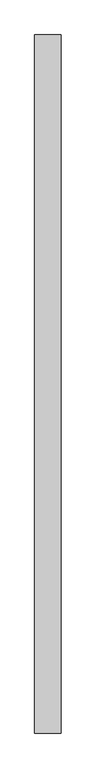
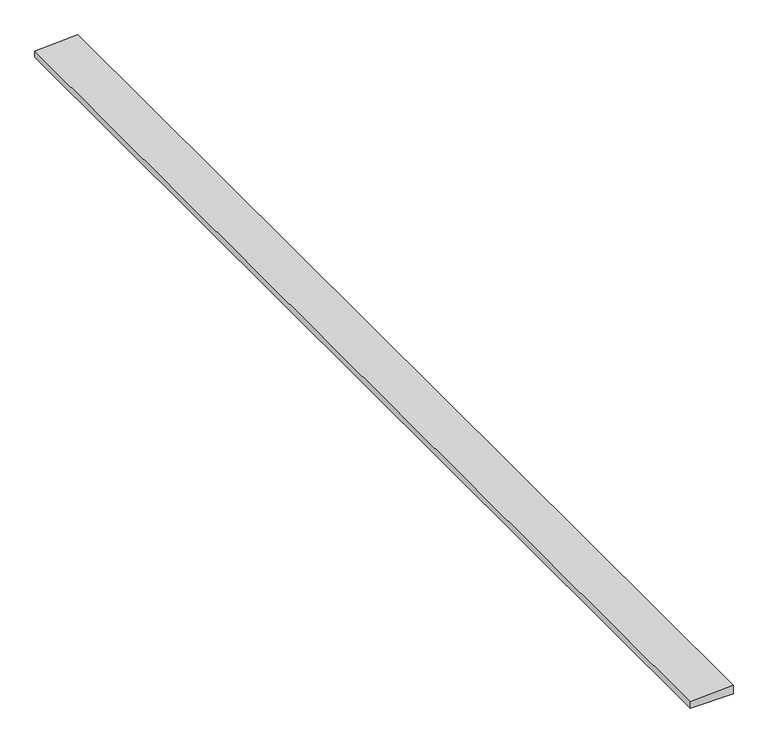
"""IFC4 building model written with IfcOpenShell, lengths in millimetres: proxy geometry, Generic Models 7:Generic Models 1:337419:Generic Models 1:337419 : Generic Models 7:Generic Models 1:337419:1 : Generic Models 7:Generic Models 1:337419:Generic Models 1:337419 : Generic Models 7:Generic Models 1:337419:301336."""

from ifc_helpers import new_model, si_unit, frame, origin, place, context, project, spatial, polyline, outline, extrude, source, transform, mapped, element, save


def generic_models_b57754ee(model_context):
    return source(origin(), model_context, "Body", "SweptSolid", [
        extrude(outline(polyline([(6130.4531764, 579296.8164664), (6168.5531764, 579296.8164664), (6158.9022838, 579112.6664664), (6130.4531764, 579112.6664664), (6130.4531764, 579296.8164664)])), frame((0.0, -578718.1163842, 0.0), z_axis=(0.0, 1.0, 0.0), x_axis=(0.0, 0.0, 1.0)), (0.0, 0.0, 1.0), 4876.8),
    ])


if __name__ == "__main__":
    model = new_model("IFC4")
    model_context = context("Model", 3, world=origin())
    ifc_project = project(units=[si_unit("LENGTHUNIT", "METRE", prefix="MILLI")], contexts=[model_context])
    site = spatial("IfcSite", under=ifc_project)
    building = spatial("IfcBuilding", under=site)
    placement = place(None, origin())
    generic_models_shape = generic_models_b57754ee(model_context)
    element("IfcBuildingElementProxy", 1, Name="Generic Models 7:Generic Models 1:337419:Generic Models 1:337419 : Generic Models 7:Generic Models 1:337419:1 : Generic Models 7:Generic Models 1:337419:Generic Models 1:337419 : Generic Models 7:Generic Models 1:337419:301336", ObjectType="Generic Models 7:Generic Models 1:337419:Generic Models 1:337419 : Generic Models 7:Generic Models 1:337419:1 : Generic Models 7:Generic Models 1:337419:Generic Models 1:337419 : Generic Models 7:Generic Models 1:337419:301336", at=placement, inside=building, context=model_context, shape_type="MappedRepresentation", body=[
        mapped(generic_models_shape, transform((0.0, 0.0, 0.0), x_axis=(1.0, 0.0, 0.0), y_axis=(0.0, 1.0, 0.0), z_axis=(0.0, 0.0, 1.0))),
    ])
    save(model, "model.ifc")

# Revit data of these elements
# Type "Generic Models 7:Generic Models 1:337419:Generic Models 1:337419 : Generic Models 7:Generic Models 1:337419:1 : Generic Models 7:Generic Models 1:337419:Generic Models 1:337419 : Generic Models 7:Generic Models 1:337419:301336"
#   NameOverride = "Generic Models 7:Generic Models 1:337419:Generic Models 1:337419 : Generic Models 7:Generic Models 1:337419:301336"
#   ObjectTypeOverride = "Generic Models 1:337419 : Generic Models 7:Generic Models 1:337419"
#   Reference = "Generic Models 1"
#   Tag = "301336"
# Element 1 (IfcBuildingElementProxy, "Generic Models 7:Generic Models 1:337419:Generic Models 1:337419 : Generic Models 7:Generic Models 1:337419:1 : Generic Models 7:Generic Models 1:337419:Generic Models 1:337419 : Generic Models 7:Generic Models 1:337419:301336")
#   Materials on its faces: "BLOCKING - SIZE AS NEC."
# Materials
#   "BLOCKING - SIZE AS NEC.": class "Wood", colour RGB 144 113 62, transparency 0, Description = "Pinus Echinata", Cost = 0
